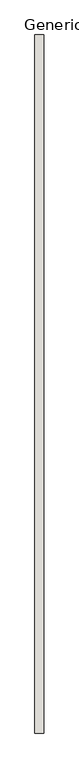
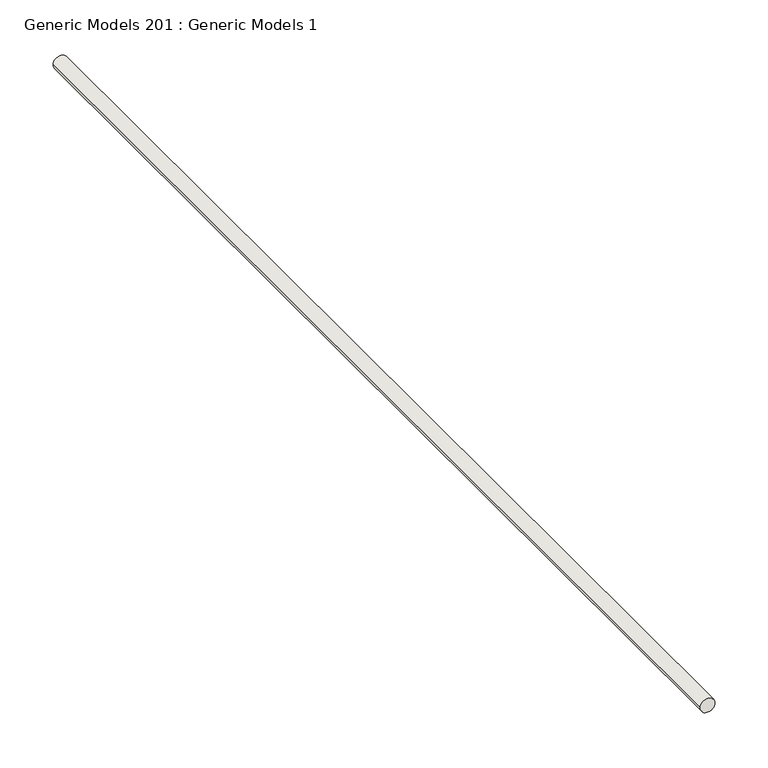
"""IFC4 building model written with IfcOpenShell, lengths in millimetres: wall geometry, Generic Models 201 : Generic Models 1."""

from ifc_helpers import new_model, si_unit, point, frame, frame_2d, origin, place, context, project, spatial, circle_curve, trimmed, segment, composite_curve, outline, extrude, source, transform, mapped, element, save


def generic_models_201_generic_models_1_de2cc35e(model_context):
    return source(origin(), model_context, "Body", "SweptSolid", [
        extrude(outline(composite_curve([segment(trimmed(circle_curve(frame_2d((2275.8814234, 748242.1328677)), 7.9375), [point((2275.8814234, 748234.1953677))], [point((2275.8814234, 748250.0703677))], False, "CARTESIAN"), True, "CONTINUOUS"), segment(trimmed(circle_curve(frame_2d((2275.8814234, 748242.1328677)), 7.9375), [point((2275.8814234, 748250.0703677))], [point((2275.8814234, 748234.1953677))], False, "CARTESIAN"), True, "CONTINUOUS")], self_intersect=False)), frame((0.0, 76.2, 0.0), z_axis=(0.0, 1.0, 0.0), x_axis=(0.0, 0.0, 1.0)), (0.0, 0.0, 1.0), 1219.2),
    ])


if __name__ == "__main__":
    model = new_model("IFC4")
    model_context = context("Model", 3, world=origin())
    ifc_project = project(units=[si_unit("LENGTHUNIT", "METRE", prefix="MILLI")], contexts=[model_context])
    site = spatial("IfcSite", under=ifc_project)
    building = spatial("IfcBuilding", under=site)
    placement = place(None, origin())
    generic_models_201_generic_models_1_shape = generic_models_201_generic_models_1_de2cc35e(model_context)
    element("IfcWall", 1, ObjectType="Generic Models 201 : Generic Models 1", at=placement, inside=building, context=model_context, shape_type="MappedRepresentation", body=[
        mapped(generic_models_201_generic_models_1_shape, transform((0.0, 0.0, 0.0), x_axis=(1.0, 0.0, 0.0), y_axis=(0.0, 1.0, 0.0), z_axis=(0.0, 0.0, 1.0))),
    ])
    save(model, "model.ifc")

# Revit data of these elements
# Element 1 (IfcWall, "Generic Models 201 : Generic Models 1")
#   Materials on its faces: "(2) #5's"
# Materials
#   "(2) #5's": class "Generic", colour RGB 255 255 255, transparency 0, Cost = 0
